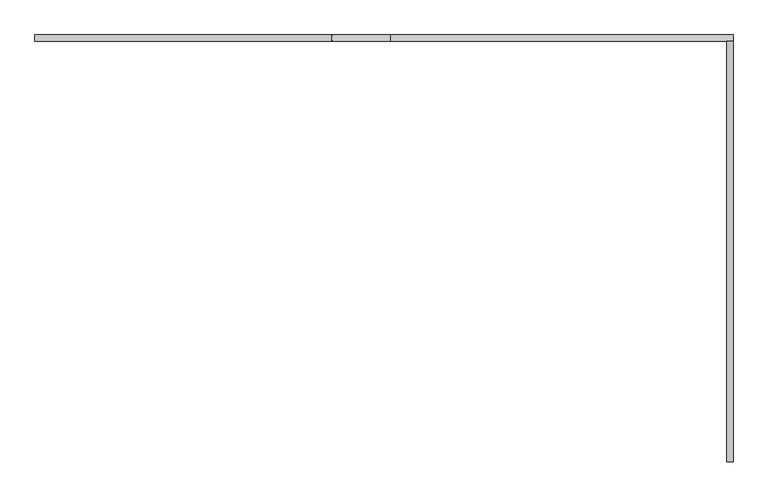
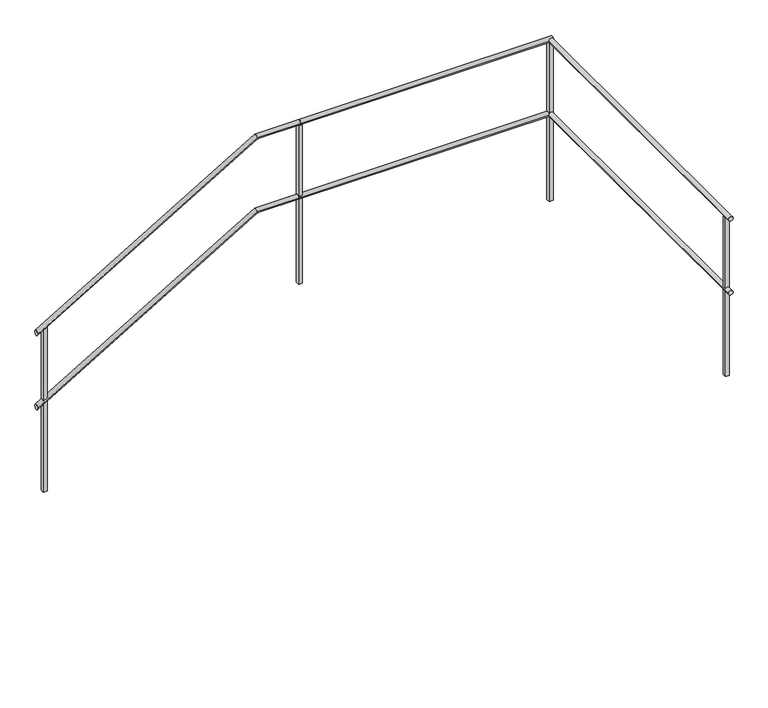
"""IFC4 building model written with IfcOpenShell, lengths in millimetres: railing geometry."""

from ifc_helpers import new_model, si_unit, frame, origin, place, context, project, spatial, polyline, circle_curve, ellipse_curve, outline, extrude, source, transform, mapped, element, save
from ifc_brep_helpers import plane_surface, cylinder_surface, advanced_brep


def railing_000ce7da(model_context):
    return source(origin(), model_context, "Body", "SolidModel", [
        advanced_brep(
        [(45466.7161135, 23749.5208589, 1734.9618634), (45496.7161135, 23749.5208589, 1734.9618634), (45466.7161135, 25734.1208589, 1734.9618634), (45496.7161135, 25734.1208589, 1734.9618634)],
        [
            (0, 1, circle_curve(frame((45481.7161135, 23749.5208589, 1734.9618634), z_axis=(0.0, -1.0, 0.0), x_axis=(1.0, 0.0, 0.0)), 15.0)),
            (1, 0, circle_curve(frame((45481.7161135, 23749.5208589, 1734.9618634), z_axis=(0.0, -1.0, 0.0), x_axis=(1.0, 0.0, 0.0)), 15.0)),
            (2, 3, circle_curve(frame((45481.7161135, 25734.1208589, 1734.9618634), z_axis=(0.0, 1.0, 0.0), x_axis=(1.0, 0.0, 0.0)), 15.0)),
            (3, 2, circle_curve(frame((45481.7161135, 25734.1208589, 1734.9618634), z_axis=(0.0, 1.0, 0.0), x_axis=(1.0, 0.0, 0.0)), 15.0)),
            (0, 2),
            (3, 1),
        ],
        [
            plane_surface(frame((45481.7161135, 23749.5208589, 1749.9618634), z_axis=(0.0, -1.0, 0.0), x_axis=(0.0, 0.0, 1.0))),
            plane_surface(frame((45481.7161135, 25734.1208589, 1749.9618634), z_axis=(0.0, 1.0, 0.0), x_axis=(0.0, 0.0, 1.0))),
            cylinder_surface(frame((45481.7161135, 23749.5208589, 1734.9618634), z_axis=(0.0, -1.0, 0.0), x_axis=(1.0, 0.0, 0.0)), 15.0),
        ],
        [
            (0, [[1, 2]]),
            (1, [[3, 4]]),
            (2, [[-1, 5, -4, 6]]),
            (2, [[-2, -6, -3, -5]]),
        ],
    ),
        advanced_brep(
        [(45496.7161135, 25734.1208589, 1734.9618634), (45496.7161135, 25764.1208589, 1734.9618634), (43882.1161135, 25734.1208589, 1734.9618634), (43882.1161135, 25764.1208589, 1734.9618634)],
        [
            (0, 1, circle_curve(frame((45496.7161135, 25749.1208589, 1734.9618634), z_axis=(1.0, 0.0, 0.0), x_axis=(0.0, 1.0, 0.0)), 15.0)),
            (1, 0, circle_curve(frame((45496.7161135, 25749.1208589, 1734.9618634), z_axis=(1.0, 0.0, 0.0), x_axis=(0.0, 1.0, 0.0)), 15.0)),
            (2, 3, circle_curve(frame((43882.1161135, 25749.1208589, 1734.9618634), z_axis=(-1.0, 0.0, 0.0), x_axis=(0.0, 1.0, 0.0)), 15.0)),
            (3, 2, circle_curve(frame((43882.1161135, 25749.1208589, 1734.9618634), z_axis=(-1.0, 0.0, 0.0), x_axis=(0.0, 1.0, 0.0)), 15.0)),
            (0, 2),
            (3, 1),
        ],
        [
            plane_surface(frame((45496.7161135, 25749.1208589, 1749.9618634), z_axis=(1.0, 0.0, 0.0), x_axis=(0.0, -1.0, 0.0))),
            plane_surface(frame((43882.1161135, 25749.1208589, 1749.9618634), z_axis=(-1.0, 0.0, 0.0), x_axis=(0.0, -1.0, 0.0))),
            cylinder_surface(frame((45496.7161135, 25749.1208589, 1734.9618634), z_axis=(1.0, 0.0, 0.0), x_axis=(0.0, 1.0, 0.0)), 15.0),
        ],
        [
            (0, [[1, 2]]),
            (1, [[3, 4]]),
            (2, [[-1, 5, -4, 6]]),
            (2, [[-2, -6, -3, -5]]),
        ],
    ),
        advanced_brep(
        [(43882.1161135, 25734.1208589, 1734.9618634), (43882.1161135, 25764.1208589, 1734.9618634), (43606.242552, 25734.1208589, 1734.9618634), (43606.242552, 25764.1208589, 1734.9618634), (42202.1161135, 25734.1208589, 899.1723166), (42202.1161135, 25764.1208589, 899.1723166)],
        [
            (0, 1, circle_curve(frame((43882.1161135, 25749.1208589, 1734.9618634), z_axis=(1.0, 0.0, 0.0), x_axis=(0.0, 1.0, 0.0)), 15.0)),
            (1, 0, circle_curve(frame((43882.1161135, 25749.1208589, 1734.9618634), z_axis=(1.0, 0.0, 0.0), x_axis=(0.0, 1.0, 0.0)), 15.0)),
            (0, 2),
            (2, 3, ellipse_curve(frame((43606.242552, 25749.1208589, 1734.9618634), z_axis=(0.9641817474962143, 0.0, 0.2652424509673111), x_axis=(0.265242450967311, 0.0, -0.9641817474962144)), 15.5572329, 15.0)),
            (3, 1),
            (3, 2, ellipse_curve(frame((43606.242552, 25749.1208589, 1734.9618634), z_axis=(0.9641817474962143, 0.0, 0.2652424509673111), x_axis=(0.265242450967311, 0.0, -0.9641817474962144)), 15.5572329, 15.0)),
            (4, 5, ellipse_curve(frame((42202.1161135, 25749.1208589, 899.1723166), z_axis=(-1.0, 0.0, 0.0), x_axis=(0.0, 0.0, 1.0)), 17.4562134, 15.0)),
            (5, 4, ellipse_curve(frame((42202.1161135, 25749.1208589, 899.1723166), z_axis=(-1.0, 0.0, 0.0), x_axis=(0.0, 0.0, 1.0)), 17.4562134, 15.0)),
            (2, 4),
            (5, 3),
        ],
        [
            plane_surface(frame((43882.1161135, 25749.1208589, 1749.9618634), z_axis=(1.0, 0.0, 0.0), x_axis=(0.0, -1.0, 0.0))),
            cylinder_surface(frame((43882.1161135, 25749.1208589, 1734.9618634), z_axis=(1.0, 0.0, 0.0), x_axis=(0.0, 1.0, 0.0)), 15.0),
            plane_surface(frame((42202.1161135, 25749.1208589, 916.62853), z_axis=(-1.0, 0.0, 0.0), x_axis=(0.0, -1.0, 0.0))),
            cylinder_surface(frame((43609.7883714, 25749.1208589, 1737.0724701), z_axis=(0.8592928844097072, 0.0, 0.5114838597676818), x_axis=(0.0, 1.0, 0.0)), 15.0),
        ],
        [
            (0, [[1, 2]]),
            (1, [[-1, 3, 4, 5]]),
            (1, [[-2, -5, 6, -3]]),
            (2, [[7, 8]]),
            (3, [[-4, 9, -8, 10]]),
            (3, [[-6, -10, -7, -9]]),
        ],
    ),
        advanced_brep(
        [(45466.7161135, 23749.5208589, 2234.9618634), (45496.7161135, 23749.5208589, 2234.9618634), (45466.7161135, 25734.1208589, 2234.9618634), (45496.7161135, 25734.1208589, 2234.9618634)],
        [
            (0, 1, circle_curve(frame((45481.7161135, 23749.5208589, 2234.9618634), z_axis=(0.0, -1.0, 0.0), x_axis=(1.0, 0.0, 0.0)), 15.0)),
            (1, 0, circle_curve(frame((45481.7161135, 23749.5208589, 2234.9618634), z_axis=(0.0, -1.0, 0.0), x_axis=(1.0, 0.0, 0.0)), 15.0)),
            (2, 3, circle_curve(frame((45481.7161135, 25734.1208589, 2234.9618634), z_axis=(0.0, 1.0, 0.0), x_axis=(1.0, 0.0, 0.0)), 15.0)),
            (3, 2, circle_curve(frame((45481.7161135, 25734.1208589, 2234.9618634), z_axis=(0.0, 1.0, 0.0), x_axis=(1.0, 0.0, 0.0)), 15.0)),
            (0, 2),
            (3, 1),
        ],
        [
            plane_surface(frame((45481.7161135, 23749.5208589, 2249.9618634), z_axis=(0.0, -1.0, 0.0), x_axis=(0.0, 0.0, 1.0))),
            plane_surface(frame((45481.7161135, 25734.1208589, 2249.9618634), z_axis=(0.0, 1.0, 0.0), x_axis=(0.0, 0.0, 1.0))),
            cylinder_surface(frame((45481.7161135, 23749.5208589, 2234.9618634), z_axis=(0.0, -1.0, 0.0), x_axis=(1.0, 0.0, 0.0)), 15.0),
        ],
        [
            (0, [[1, 2]]),
            (1, [[3, 4]]),
            (2, [[-1, 5, -4, 6]]),
            (2, [[-2, -6, -3, -5]]),
        ],
    ),
        advanced_brep(
        [(45496.7161135, 25734.1208589, 2234.9618634), (45496.7161135, 25764.1208589, 2234.9618634), (43882.1161135, 25734.1208589, 2234.9618634), (43882.1161135, 25764.1208589, 2234.9618634)],
        [
            (0, 1, circle_curve(frame((45496.7161135, 25749.1208589, 2234.9618634), z_axis=(1.0, 0.0, 0.0), x_axis=(0.0, 1.0, 0.0)), 15.0)),
            (1, 0, circle_curve(frame((45496.7161135, 25749.1208589, 2234.9618634), z_axis=(1.0, 0.0, 0.0), x_axis=(0.0, 1.0, 0.0)), 15.0)),
            (2, 3, circle_curve(frame((43882.1161135, 25749.1208589, 2234.9618634), z_axis=(-1.0, 0.0, 0.0), x_axis=(0.0, 1.0, 0.0)), 15.0)),
            (3, 2, circle_curve(frame((43882.1161135, 25749.1208589, 2234.9618634), z_axis=(-1.0, 0.0, 0.0), x_axis=(0.0, 1.0, 0.0)), 15.0)),
            (0, 2),
            (3, 1),
        ],
        [
            plane_surface(frame((45496.7161135, 25749.1208589, 2249.9618634), z_axis=(1.0, 0.0, 0.0), x_axis=(0.0, -1.0, 0.0))),
            plane_surface(frame((43882.1161135, 25749.1208589, 2249.9618634), z_axis=(-1.0, 0.0, 0.0), x_axis=(0.0, -1.0, 0.0))),
            cylinder_surface(frame((45496.7161135, 25749.1208589, 2234.9618634), z_axis=(1.0, 0.0, 0.0), x_axis=(0.0, 1.0, 0.0)), 15.0),
        ],
        [
            (0, [[1, 2]]),
            (1, [[3, 4]]),
            (2, [[-1, 5, -4, 6]]),
            (2, [[-2, -6, -3, -5]]),
        ],
    ),
        advanced_brep(
        [(43882.1161135, 25734.1208589, 2234.9618634), (43882.1161135, 25764.1208589, 2234.9618634), (43606.242552, 25734.1208589, 2234.9618634), (43606.242552, 25764.1208589, 2234.9618634), (42202.1161135, 25734.1208589, 1399.1723166), (42202.1161135, 25764.1208589, 1399.1723166)],
        [
            (0, 1, circle_curve(frame((43882.1161135, 25749.1208589, 2234.9618634), z_axis=(1.0, 0.0, 0.0), x_axis=(0.0, 1.0, 0.0)), 15.0)),
            (1, 0, circle_curve(frame((43882.1161135, 25749.1208589, 2234.9618634), z_axis=(1.0, 0.0, 0.0), x_axis=(0.0, 1.0, 0.0)), 15.0)),
            (0, 2),
            (2, 3, ellipse_curve(frame((43606.242552, 25749.1208589, 2234.9618634), z_axis=(0.9641817474962143, 0.0, 0.2652424509673111), x_axis=(0.265242450967311, 0.0, -0.9641817474962144)), 15.5572329, 15.0)),
            (3, 1),
            (3, 2, ellipse_curve(frame((43606.242552, 25749.1208589, 2234.9618634), z_axis=(0.9641817474962143, 0.0, 0.2652424509673111), x_axis=(0.265242450967311, 0.0, -0.9641817474962144)), 15.5572329, 15.0)),
            (4, 5, ellipse_curve(frame((42202.1161135, 25749.1208589, 1399.1723166), z_axis=(-1.0, 0.0, 0.0), x_axis=(0.0, 0.0, 1.0)), 17.4562134, 15.0)),
            (5, 4, ellipse_curve(frame((42202.1161135, 25749.1208589, 1399.1723166), z_axis=(-1.0, 0.0, 0.0), x_axis=(0.0, 0.0, 1.0)), 17.4562134, 15.0)),
            (2, 4),
            (5, 3),
        ],
        [
            plane_surface(frame((43882.1161135, 25749.1208589, 2249.9618634), z_axis=(1.0, 0.0, 0.0), x_axis=(0.0, -1.0, 0.0))),
            cylinder_surface(frame((43882.1161135, 25749.1208589, 2234.9618634), z_axis=(1.0, 0.0, 0.0), x_axis=(0.0, 1.0, 0.0)), 15.0),
            plane_surface(frame((42202.1161135, 25749.1208589, 1416.62853), z_axis=(-1.0, 0.0, 0.0), x_axis=(0.0, -1.0, 0.0))),
            cylinder_surface(frame((43609.7883714, 25749.1208589, 2237.0724701), z_axis=(0.8592928844097072, 0.0, 0.5114838597676818), x_axis=(0.0, 1.0, 0.0)), 15.0),
        ],
        [
            (0, [[1, 2]]),
            (1, [[-1, 3, 4, 5]]),
            (1, [[-2, -5, 6, -3]]),
            (2, [[7, 8]]),
            (3, [[-4, 9, -8, 10]]),
            (3, [[-6, -10, -7, -9]]),
        ],
    ),
        extrude(outline(polyline([(43894.6161135, 25761.6208589), (43894.6161135, 25736.6208589), (43869.6161135, 25736.6208589), (43869.6161135, 25761.6208589), (43894.6161135, 25761.6208589)])), frame((0.0, 0.0, 1149.9618634), z_axis=(0.0, 0.0, 1.0), x_axis=(1.0, 0.0, 0.0)), (0.0, 0.0, 1.0), 1070.0),
        extrude(outline(polyline([(45494.2161135, 25736.6208589), (45469.2161135, 25736.6208589), (45469.2161135, 25761.6208589), (45494.2161135, 25761.6208589), (45494.2161135, 25736.6208589)])), frame((0.0, 0.0, 1149.9618634), z_axis=(0.0, 0.0, 1.0), x_axis=(1.0, 0.0, 0.0)), (0.0, 0.0, 1.0), 1070.0),
        extrude(outline(polyline([(316.62853, 42264.6161135), (1423.830911, 42264.6161135), (1408.9499586, 42239.6161135), (316.62853, 42239.6161135), (316.62853, 42264.6161135)])), frame((0.0, 25736.6208589, 0.0), z_axis=(0.0, 1.0, 0.0), x_axis=(0.0, 0.0, 1.0)), (0.0, 0.0, 1.0), 25.0),
        extrude(outline(polyline([(45494.2161135, 23787.0208589), (45469.2161135, 23787.0208589), (45469.2161135, 23812.0208589), (45494.2161135, 23812.0208589), (45494.2161135, 23787.0208589)])), frame((0.0, 0.0, 1149.9618634), z_axis=(0.0, 0.0, 1.0), x_axis=(1.0, 0.0, 0.0)), (0.0, 0.0, 1.0), 1070.0),
    ])


if __name__ == "__main__":
    model = new_model("IFC4")
    model_context = context("Model", 3, world=origin())
    ifc_project = project(units=[si_unit("LENGTHUNIT", "METRE", prefix="MILLI")], contexts=[model_context])
    site = spatial("IfcSite", under=ifc_project)
    building = spatial("IfcBuilding", under=site)
    placement = place(None, origin())
    railing_shape = railing_000ce7da(model_context)
    element("IfcRailing", 1, at=placement, inside=building, context=model_context, shape_type="MappedRepresentation", body=[
        mapped(railing_shape, transform((0.0, 0.0, 0.0), x_axis=(1.0, 0.0, 0.0), y_axis=(0.0, 1.0, 0.0), z_axis=(0.0, 0.0, 1.0))),
    ])
    save(model, "model.ifc")
